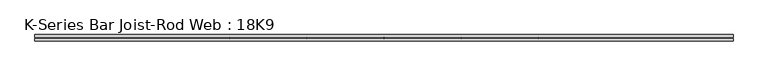
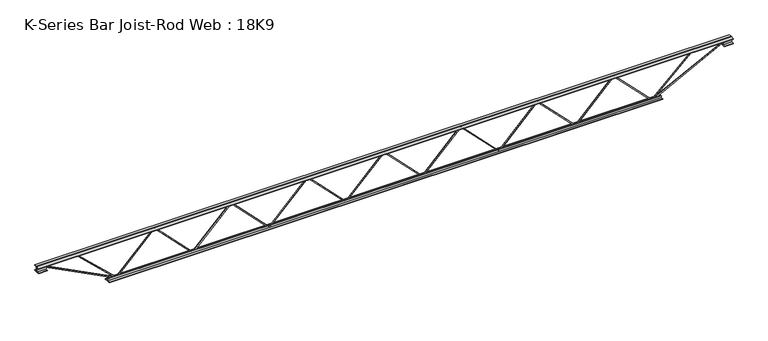
"""IFC4 building model written with IfcOpenShell, lengths in millimetres: beam geometry, K-Series Bar Joist-Rod Web : 18K9."""

from ifc_helpers import new_model, si_unit, frame, origin, place, context, project, spatial, polyline, outline, extrude, source, transform, mapped, element, save


def k_series_bar_joist_rod_web_18k9_06ccdaad(model_context):
    return source(origin(), model_context, "Body", "SweptSolid", [
        extrude(outline(polyline([(-217.4875, 1323.2946429), (-227.0125, 1323.2946429), (-227.0125, 1328.4733471), (217.4875, 1763.2215614), (217.4875, 1765.5641529), (-227.0125, 2200.3123672), (-227.0125, 2205.4910714), (-217.4875, 2205.4910714), (-217.4875, 2204.3197757), (227.0125, 1769.5715614), (227.0125, 1759.2141529), (-217.4875, 1324.4659386), (-217.4875, 1323.2946429)])), frame((0.0, -4.7625, 0.0), z_axis=(0.0, 1.0, 0.0), x_axis=(0.0, 0.0, 1.0)), (0.0, 0.0, 1.0), 9.525),
        extrude(outline(polyline([(-217.4875, 441.0982143), (-227.0125, 441.0982143), (-227.0125, 446.2769186), (217.4875, 881.0251328), (217.4875, 883.3677243), (-227.0125, 1318.1159386), (-227.0125, 1323.2946429), (-217.4875, 1323.2946429), (-217.4875, 1322.1233471), (227.0125, 887.3751328), (227.0125, 877.0177243), (-217.4875, 442.26951), (-217.4875, 441.0982143)])), frame((0.0, -4.7625, 0.0), z_axis=(0.0, 1.0, 0.0), x_axis=(0.0, 0.0, 1.0)), (0.0, 0.0, 1.0), 9.525),
        extrude(outline(polyline([(-217.4875, -441.0982143), (-227.0125, -441.0982143), (-227.0125, -435.91951), (217.4875, -1.1712957), (217.4875, 1.1712957), (-227.0125, 435.91951), (-227.0125, 441.0982143), (-217.4875, 441.0982143), (-217.4875, 439.9269186), (227.0125, 5.1787043), (227.0125, -5.1787043), (-217.4875, -439.9269186), (-217.4875, -441.0982143)])), frame((0.0, -4.7625, 0.0), z_axis=(0.0, 1.0, 0.0), x_axis=(0.0, 0.0, 1.0)), (0.0, 0.0, 1.0), 9.525),
        extrude(outline(polyline([(-217.4875, -1323.2946429), (-227.0125, -1323.2946429), (-227.0125, -1318.1159386), (217.4875, -883.3677243), (217.4875, -881.0251328), (-227.0125, -446.2769186), (-227.0125, -441.0982143), (-217.4875, -441.0982143), (-217.4875, -442.26951), (227.0125, -877.0177243), (227.0125, -887.3751328), (-217.4875, -1322.1233471), (-217.4875, -1323.2946429)])), frame((0.0, -4.7625, 0.0), z_axis=(0.0, 1.0, 0.0), x_axis=(0.0, 0.0, 1.0)), (0.0, 0.0, 1.0), 9.525),
        extrude(outline(polyline([(-217.4875, -2205.4910714), (-227.0125, -2205.4910714), (-227.0125, -2200.3123672), (217.4875, -1765.5641529), (217.4875, -1763.2215614), (-227.0125, -1328.4733471), (-227.0125, -1323.2946429), (-217.4875, -1323.2946429), (-217.4875, -1324.4659386), (227.0125, -1759.2141529), (227.0125, -1769.5715614), (-217.4875, -2204.3197757), (-217.4875, -2205.4910714)])), frame((0.0, -4.7625, 0.0), z_axis=(0.0, 1.0, 0.0), x_axis=(0.0, 0.0, 1.0)), (0.0, 0.0, 1.0), 9.525),
        extrude(outline(polyline([(-217.4875, 2205.4910714), (-227.0125, 2205.4910714), (-227.0125, 2210.6697757), (217.4875, 2645.41799), (217.4875, 2647.7605814), (-227.0125, 3082.5087957), (-227.0125, 3087.6875), (-217.4875, 3087.6875), (-217.4875, 3086.5162043), (227.0125, 2651.76799), (227.0125, 2641.4105814), (-217.4875, 2206.6623672), (-217.4875, 2205.4910714)])), frame((0.0, -4.7625, 0.0), z_axis=(0.0, 1.0, 0.0), x_axis=(0.0, 0.0, 1.0)), (0.0, 0.0, 1.0), 9.525),
        extrude(outline(polyline([(-217.4875, -3087.6875), (-227.0125, -3087.6875), (-227.0125, -3082.5087957), (217.4875, -2647.7605814), (217.4875, -2645.41799), (-227.0125, -2210.6697757), (-227.0125, -2205.4910714), (-217.4875, -2205.4910714), (-217.4875, -2206.6623672), (227.0125, -2641.4105814), (227.0125, -2651.76799), (-217.4875, -3086.5162043), (-217.4875, -3087.6875)])), frame((0.0, -4.7625, 0.0), z_axis=(0.0, 1.0, 0.0), x_axis=(0.0, 0.0, 1.0)), (0.0, 0.0, 1.0), 9.525),
        extrude(outline(polyline([(4.7625, 228.6), (36.5125, 228.6), (36.5125, 222.25), (11.1125, 222.25), (11.1125, 196.85), (4.7625, 196.85), (4.7625, 228.6)])), frame((-4002.0875, 0.0, 0.0), z_axis=(1.0, 0.0, 0.0), x_axis=(0.0, 1.0, 0.0)), (0.0, 0.0, 1.0), 8004.175),
        extrude(outline(polyline([(-4.7625, 228.6), (-4.7625, 196.85), (-11.1125, 196.85), (-11.1125, 222.25), (-36.5125, 222.25), (-36.5125, 228.6), (-4.7625, 228.6)])), frame((-4002.0875, 0.0, 0.0), z_axis=(1.0, 0.0, 0.0), x_axis=(0.0, 1.0, 0.0)), (0.0, 0.0, 1.0), 8004.175),
        extrude(outline(polyline([(-4.7625, 165.1), (-36.5125, 165.1), (-36.5125, 171.45), (-11.1125, 171.45), (-11.1125, 196.85), (-4.7625, 196.85), (-4.7625, 165.1)])), frame((-4002.0875, 0.0, 0.0), z_axis=(1.0, 0.0, 0.0), x_axis=(0.0, 1.0, 0.0)), (0.0, 0.0, 1.0), 101.6),
        extrude(outline(polyline([(36.5125, 165.1), (4.7625, 165.1), (4.7625, 196.85), (11.1125, 196.85), (11.1125, 171.45), (36.5125, 171.45), (36.5125, 165.1)])), frame((-4002.0875, 0.0, 0.0), z_axis=(1.0, 0.0, 0.0), x_axis=(0.0, 1.0, 0.0)), (0.0, 0.0, 1.0), 101.6),
        extrude(outline(polyline([(4.7625, 165.1), (4.7625, 196.85), (11.1125, 196.85), (11.1125, 171.45), (36.5125, 171.45), (36.5125, 165.1), (4.7625, 165.1)])), frame((3900.4875, 0.0, 0.0), z_axis=(1.0, 0.0, 0.0), x_axis=(0.0, 1.0, 0.0)), (0.0, 0.0, 1.0), 101.6),
        extrude(outline(polyline([(-4.7625, 165.1), (-36.5125, 165.1), (-36.5125, 171.45), (-11.1125, 171.45), (-11.1125, 196.85), (-4.7625, 196.85), (-4.7625, 165.1)])), frame((3900.4875, 0.0, 0.0), z_axis=(1.0, 0.0, 0.0), x_axis=(0.0, 1.0, 0.0)), (0.0, 0.0, 1.0), 101.6),
        extrude(outline(polyline([(4.7625, -228.6), (4.7625, -196.85), (11.1125, -196.85), (11.1125, -222.25), (36.5125, -222.25), (36.5125, -228.6), (4.7625, -228.6)])), frame((-3189.2875, 0.0, 0.0), z_axis=(1.0, 0.0, 0.0), x_axis=(0.0, 1.0, 0.0)), (0.0, 0.0, 1.0), 6378.575),
        extrude(outline(polyline([(-4.7625, -228.6), (-36.5125, -228.6), (-36.5125, -222.25), (-11.1125, -222.25), (-11.1125, -196.85), (-4.7625, -196.85), (-4.7625, -228.6)])), frame((-3189.2875, 0.0, 0.0), z_axis=(1.0, 0.0, 0.0), x_axis=(0.0, 1.0, 0.0)), (0.0, 0.0, 1.0), 6378.575),
        extrude(outline(polyline([(0.0, -9.525), (0.0, 0.0), (914.4881902, 0.0), (914.4881902, -9.525), (0.0, -9.525)])), frame((-3902.670102, 4.7625, 192.6170749), z_axis=(0.45828913319472714, 0.0, 0.8888031674086371), x_axis=(0.8888031674086371, 0.0, -0.45828913319472714)), (0.0, 0.0, 1.0), 9.525),
        extrude(outline(polyline([(0.0, -9.525), (0.0, 0.0), (608.4508564, 0.0), (608.4508564, -9.525), (0.0, -9.525)])), frame((-3532.0661169, 4.7625, 193.3974118), z_axis=(0.6887984388483902, 0.0, 0.7249529023598847), x_axis=(0.7249529023598847, 0.0, -0.6887984388483902)), (0.0, 0.0, 1.0), 9.525),
        extrude(outline(polyline([(0.0, -9.525), (0.0, 0.0), (914.4881902, 0.0), (914.4881902, -9.525), (0.0, -9.525)])), frame((3902.670102, -4.7625, 192.6170749), z_axis=(-0.4582891331947156, 0.0, 0.8888031674086431), x_axis=(-0.8888031674086431, 0.0, -0.4582891331947156)), (0.0, 0.0, 1.0), 9.525),
        extrude(outline(polyline([(0.0, -9.525), (0.0, 0.0), (608.4508564, 0.0), (608.4508564, -9.525), (0.0, -9.525)])), frame((3532.0661169, -4.7625, 193.3974118), z_axis=(-0.6887984388483861, 0.0, 0.7249529023598885), x_axis=(-0.7249529023598885, 0.0, -0.6887984388483861)), (0.0, 0.0, 1.0), 9.525),
    ])


if __name__ == "__main__":
    model = new_model("IFC4")
    model_context = context("Model", 3, world=origin())
    ifc_project = project(units=[si_unit("LENGTHUNIT", "METRE", prefix="MILLI")], contexts=[model_context])
    site = spatial("IfcSite", under=ifc_project)
    building = spatial("IfcBuilding", under=site)
    placement = place(None, origin())
    k_series_bar_joist_rod_web_18k9_shape = k_series_bar_joist_rod_web_18k9_06ccdaad(model_context)
    element("IfcBeam", 1, ObjectType="K-Series Bar Joist-Rod Web : 18K9", at=placement, inside=building, context=model_context, shape_type="MappedRepresentation", body=[
        mapped(k_series_bar_joist_rod_web_18k9_shape, transform((0.0, 0.0, 0.0), x_axis=(1.0, 0.0, 0.0), y_axis=(0.0, 1.0, 0.0), z_axis=(0.0, 0.0, 1.0))),
    ])
    save(model, "model.ifc")

# Revit data of these elements
# Type "K-Series Bar Joist-Rod Web : 18K9"
#   Assembly Code = "B1010350"
#   Wt = 10.2
#   Web Thickness = 0' - 0 3/8"
#   Start Offset [instance default] = 0' - 0"
#   Start Extension [instance default] = 0' - 0"
#   Seat Length = 0' - 4"
#   Seat Depth = 0' - 2 1/2"
#   PanelArrayLength [instance default] = 18' - 0"
#   Panel [instance default] = 3' - 0"
#   End Offset [instance default] = 0' - 0"
#   End Extension [instance default] = 0' - 0"
#   End Panel = 3' - 0"
#   Cord Leg = 0' - 1 1/4"
#   Chord Thickness = 0' - 0 1/4"
#   Length [instance default] = 24' - 0"
#   Depth = 1' - 6"
#   PanelArrayNum [instance default] = 6
#   Structural Material = none
# Element 1 (IfcBeam, "K-Series Bar Joist-Rod Web : 18K9")
#   PanelArrayLength = 20' - 3 1/8"
#   Panel = 2' - 10.73214"
#   PanelArrayNum = 7
